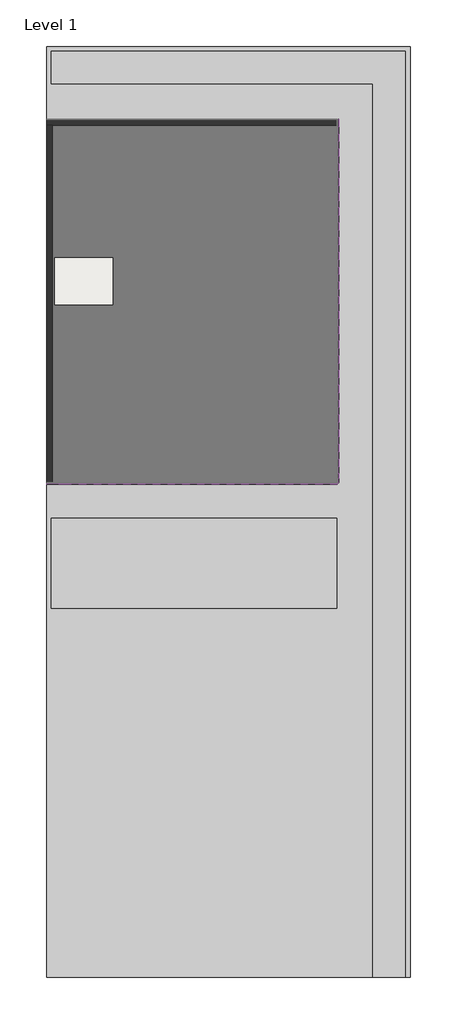
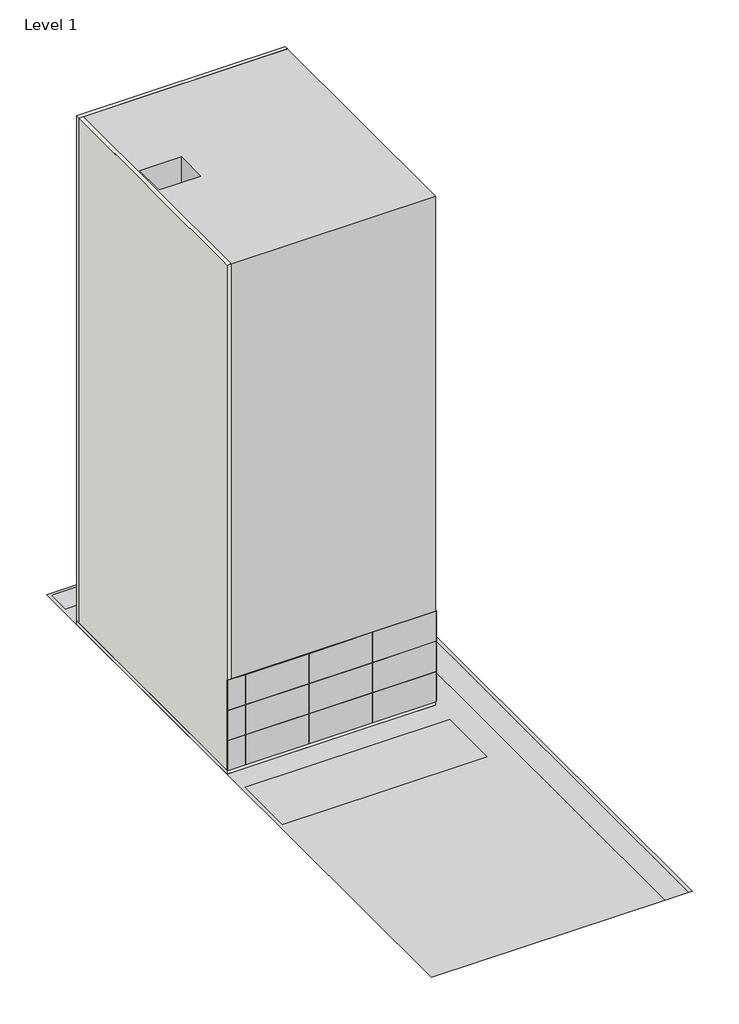
# One storey: 27 plates, 4 proxies, 2 walls, 1 slab.
"""IFC4 building model written with IfcOpenShell, lengths in millimetres."""

import ifcopenshell
import ifcopenshell.guid

model = None  # the IFC model being written
_history = None  # IfcOwnerHistory: only IFC2X3 demands one
_inside = {}  # id of a spatial element -> (the spatial element, [elements in it])
_under = {}  # id of a project, library or spatial element -> (it, [spatial elements below it])
_declared = {}  # id of a project -> (the project, [libraries it declares])
_typed = {}  # id of a type object -> (the type object, [elements of that type])
_made_of = {}  # id of a material, layer set ... -> (it, [elements and type objects made of it])


def new_model(schema):
    """Start an empty IFC model of exactly this schema.

    Asked for "IFC4X3", IfcOpenShell would pick the latest addendum, in which some entities
    have other attributes; the version numbers below select the first issue.
    IFC2X3 requires an IfcOwnerHistory on every rooted entity: one is made here for all.
    """
    global model, _history
    if schema == "IFC4X3":
        model = ifcopenshell.file(schema_version=(4, 3, 0, 0))
    else:
        model = ifcopenshell.file(schema=schema)
    _inside.clear()
    _under.clear()
    _declared.clear()
    _typed.clear()
    _made_of.clear()
    _history = None
    if model.schema == "IFC2X3":
        org = make("IfcOrganization", Name="unknown")
        user = make(
            "IfcPersonAndOrganization",
            ThePerson=make("IfcPerson", FamilyName="unknown"),
            TheOrganization=org,
        )
        app = make(
            "IfcApplication",
            ApplicationDeveloper=org,
            Version="unknown",
            ApplicationFullName="unknown",
            ApplicationIdentifier="unknown",
        )
        _history = make(
            "IfcOwnerHistory",
            OwningUser=user,
            OwningApplication=app,
            ChangeAction="ADDED",
            CreationDate=0,
        )
    return model


def make(cls, **values):
    """One entity of the class cls with the attributes given. An attribute that is None is left unset."""
    return model.create_entity(
        cls, **{name: value for name, value in values.items() if value is not None}
    )


def rooted(cls, **values):
    """An entity with a GlobalId (a new one), such as an element, a storey or a relation."""
    return make(cls, GlobalId=ifcopenshell.guid.new(), OwnerHistory=_history, **values)


def si_unit(unit_type, name, prefix=None):
    """IfcSIUnit, for example si_unit("LENGTHUNIT", "METRE", prefix="MILLI")."""
    return make("IfcSIUnit", UnitType=unit_type, Prefix=prefix, Name=name)


def assignment(units):
    """IfcUnitAssignment: the units of a project."""
    return None if units is None else make("IfcUnitAssignment", Units=units)


def point(xyz):
    """IfcCartesianPoint."""
    return None if xyz is None else make("IfcCartesianPoint", Coordinates=xyz)


def direction(xyz):
    """IfcDirection."""
    return None if xyz is None else make("IfcDirection", DirectionRatios=xyz)


def frame(location, z_axis=None, x_axis=None):
    """IfcAxis2Placement3D, a coordinate frame: its origin and axes. An axis left out is left unset."""
    return make(
        "IfcAxis2Placement3D",
        Location=point(location),
        Axis=direction(z_axis),
        RefDirection=direction(x_axis),
    )


def origin():
    """The frame at (0, 0, 0) with its axes left unset."""
    return frame((0.0, 0.0, 0.0))


def origin_with_axes():
    """The frame at (0, 0, 0) with the z axis (0, 0, 1) and the x axis (1, 0, 0) written out."""
    return frame((0.0, 0.0, 0.0), z_axis=(0.0, 0.0, 1.0), x_axis=(1.0, 0.0, 0.0))


def place(relative_to, where):
    """IfcLocalPlacement: puts the frame where relative to a parent placement (None: the world)."""
    return make(
        "IfcLocalPlacement", PlacementRelTo=relative_to, RelativePlacement=where
    )


def context(
    kind, dimensions, precision=None, world=None, true_north=None, identifier=None
):
    """IfcGeometricRepresentationContext, for example the 3D "Model" context."""
    return make(
        "IfcGeometricRepresentationContext",
        ContextIdentifier=identifier,
        ContextType=kind,
        CoordinateSpaceDimension=dimensions,
        Precision=precision,
        WorldCoordinateSystem=world,
        TrueNorth=true_north,
    )


def project(units=None, contexts=None):
    """IfcProject with its units and contexts."""
    return rooted(
        "IfcProject",
        Name="project",
        RepresentationContexts=contexts,
        UnitsInContext=assignment(units),
    )


def spatial(cls, under=None, at=None, **own):
    """A site, building, storey or space (cls), placed at a placement, below another one or the project."""
    s = rooted(cls, ObjectPlacement=at, **own)
    if under is not None:
        _under.setdefault(under.id(), (under, []))[1].append(s)
    return s


def polyline(points):
    """IfcPolyline through the points."""
    return make("IfcPolyline", Points=[point(p) for p in points])


def point_list(points):
    """IfcCartesianPointList2D or 3D."""
    cls = (
        "IfcCartesianPointList2D" if len(points[0]) == 2 else "IfcCartesianPointList3D"
    )
    return make(cls, CoordList=points)


def outline(outer, holes=None, kind="AREA"):
    """IfcArbitraryClosedProfileDef: a profile drawn as a closed curve; with holes, ...WithVoids."""
    if holes is None:
        return make("IfcArbitraryClosedProfileDef", ProfileType=kind, OuterCurve=outer)
    return make(
        "IfcArbitraryProfileDefWithVoids",
        ProfileType=kind,
        OuterCurve=outer,
        InnerCurves=holes,
    )


def extrude(swept, where, along, depth):
    """IfcExtrudedAreaSolid: the profile swept, set in the frame where, extruded along a direction by depth."""
    return make(
        "IfcExtrudedAreaSolid",
        SweptArea=swept,
        Position=where,
        ExtrudedDirection=direction(along),
        Depth=depth,
    )


def faces_of(points, faces, orient=None, outer=None):
    """IfcFace entities. A face is a list of loops; a loop is a list of indices into points, from 0.

    orient and outer hold one flag for each loop. By default every Orientation is true, the
    first loop of a face is its IfcFaceOuterBound and the others are IfcFaceBound.
    """
    made = []
    for i, loops in enumerate(faces):
        bounds = []
        for j, loop in enumerate(loops):
            is_outer = j == 0 if outer is None else outer[i][j]
            bounds.append(
                make(
                    "IfcFaceOuterBound" if is_outer else "IfcFaceBound",
                    Bound=make("IfcPolyLoop", Polygon=[points[k] for k in loop]),
                    Orientation=True if orient is None else orient[i][j],
                )
            )
        made.append(make("IfcFace", Bounds=bounds))
    return made


def faceted_brep(points, faces, orient=None, outer=None, voids=None):
    """IfcFacetedBrep: a solid bounded by flat faces; with voids (closed shells), ...WithVoids."""
    shared = [point(p) for p in points]
    hull = make("IfcClosedShell", CfsFaces=faces_of(shared, faces, orient, outer))
    if voids is None:
        return make("IfcFacetedBrep", Outer=hull)
    return make(
        "IfcFacetedBrepWithVoids",
        Outer=hull,
        Voids=[
            make(cls, CfsFaces=faces_of(shared, fs, o, b)) for cls, fs, o, b in voids
        ],
    )


def triangles(points, corners, closed=None, point_numbers=None):
    """IfcTriangulatedFaceSet: each triangle names its three corners, points numbered from 1."""
    return make(
        "IfcTriangulatedFaceSet",
        Coordinates=point_list(points),
        Closed=closed,
        CoordIndex=corners,
        PnIndex=point_numbers,
    )


def shape(context_of_items, identifier, shape_type, items):
    """IfcShapeRepresentation: the items that make up one representation, for example the "Body"."""
    return make(
        "IfcShapeRepresentation",
        ContextOfItems=context_of_items,
        RepresentationIdentifier=identifier,
        RepresentationType=shape_type,
        Items=items,
    )


def source(mapping_origin, context_of_items, identifier, shape_type, items):
    """IfcRepresentationMap: a shape defined once, which mapped items show again and again."""
    return make(
        "IfcRepresentationMap",
        MappingOrigin=mapping_origin,
        MappedRepresentation=shape(context_of_items, identifier, shape_type, items),
    )


def transform(
    local_origin,
    x_axis=None,
    y_axis=None,
    z_axis=None,
    scale=None,
    scale2=None,
    scale3=None,
    uniform=True,
):
    """IfcCartesianTransformationOperator3D, or its non-uniform kind. x_axis, y_axis, z_axis: its Axis1, 2, 3."""
    if uniform:
        return make(
            "IfcCartesianTransformationOperator3D",
            Axis1=direction(x_axis),
            Axis2=direction(y_axis),
            LocalOrigin=point(local_origin),
            Scale=scale,
            Axis3=direction(z_axis),
        )
    return make(
        "IfcCartesianTransformationOperator3DnonUniform",
        Axis1=direction(x_axis),
        Axis2=direction(y_axis),
        LocalOrigin=point(local_origin),
        Scale=scale,
        Axis3=direction(z_axis),
        Scale2=scale2,
        Scale3=scale3,
    )


def mapped(mapping_source, mapping_target):
    """IfcMappedItem: shows the shape of a source again, moved by a transform."""
    return make(
        "IfcMappedItem", MappingSource=mapping_source, MappingTarget=mapping_target
    )


def made_of(thing, what):
    """Note that an element or type object is made of a material, layer set ...; save() writes the relation."""
    if what is not None:
        _made_of.setdefault(what.id(), (what, []))[1].append(thing)
    return thing


def element(
    cls,
    number,
    at=None,
    inside=None,
    cuts=None,
    type_object=None,
    material=None,
    context=None,
    identifier="Body",
    shape_type=None,
    held_by="IfcProductDefinitionShape",
    body=None,
    shapes=None,
    **own,
):
    """One element of the class cls, such as IfcWall. Its Tag is "e" and its number.

    at: its placement. inside: the storey or other place that contains it. cuts: it is an
    opening in that element (IfcRelVoidsElement). A single representation is given by context,
    identifier, shape_type and body (its items); several are given by shapes. held_by: the class
    of the entity that holds the representations. save() writes the other relations.
    """
    e = rooted(cls, Tag="e%d" % number, ObjectPlacement=at, **own)
    if body is not None:
        shapes = [shape(context, identifier, shape_type, body)]
    if shapes is not None:
        e.Representation = make(held_by, Representations=shapes)
    if inside is not None:
        _inside.setdefault(inside.id(), (inside, []))[1].append(e)
    if cuts is not None:
        rooted(
            "IfcRelVoidsElement", RelatingBuildingElement=cuts, RelatedOpeningElement=e
        )
    if type_object is not None:
        _typed.setdefault(type_object.id(), (type_object, []))[1].append(e)
    return made_of(e, material)


def aggregate(whole, parts):
    """IfcRelAggregates: a whole, such as a stair, and the parts it consists of."""
    return rooted("IfcRelAggregates", RelatingObject=whole, RelatedObjects=parts)


def save(model, path):
    """Write the relations noted so far, then the file.

    IfcRelAggregates (storeys below a building ...), IfcRelContainedInSpatialStructure (elements
    in a storey), IfcRelDefinesByType, IfcRelAssociatesMaterial and IfcRelDeclares: one each for
    every whole, place, type object, material and project.
    """
    for whole, parts in _under.values():
        aggregate(whole, parts)
    for where, things in _inside.values():
        rooted(
            "IfcRelContainedInSpatialStructure",
            RelatedElements=things,
            RelatingStructure=where,
        )
    for kind, things in _typed.values():
        rooted("IfcRelDefinesByType", RelatedObjects=things, RelatingType=kind)
    for what, things in _made_of.values():
        rooted("IfcRelAssociatesMaterial", RelatedObjects=things, RelatingMaterial=what)
    for by, libraries in _declared.values():
        rooted("IfcRelDeclares", RelatingContext=by, RelatedDefinitions=libraries)
    model.write(path)


def system_panel_glazed_1e57f9bb(model_context):
    return source(origin(), model_context, "Body", "SweptSolid", [
        extrude(outline(polyline([(1524.0000002, 19.05), (-1524.0000002, 19.05), (-1524.0000002, 44.45), (1524.0000002, 44.45), (1524.0000002, 19.05)])), origin_with_axes(), (0.0, 0.0, 1.0), 1524.0),
    ])


def system_panel_glazed_ccfd9adb(model_context):
    return source(origin(), model_context, "Body", "SweptSolid", [
        extrude(outline(polyline([(427.9999998, 19.05), (-427.9999998, 19.05), (-427.9999998, 44.45), (427.9999998, 44.45), (427.9999998, 19.05)])), origin_with_axes(), (0.0, 0.0, 1.0), 1524.0),
    ])


def system_panel_glazed_88f24eba(model_context):
    return source(origin(), model_context, "Body", "SweptSolid", [
        extrude(outline(polyline([(153.9999998, 19.05), (-153.9999998, 19.05), (-153.9999998, 44.45), (153.9999998, 44.45), (153.9999998, 19.05)])), origin_with_axes(), (0.0, 0.0, 1.0), 1524.0),
    ])


model = new_model("IFC4")

# Units and contexts
model_context = context("Model", 3, world=origin())
ifc_project = project(units=[si_unit("LENGTHUNIT", "METRE", prefix="MILLI")], contexts=[model_context])

# Site, building, storey
site = spatial("IfcSite", under=ifc_project)
building = spatial("IfcBuilding", under=site)
storey = spatial("IfcBuildingStorey", under=building, Name="Level 1", Elevation=0.0)

# Proxies
placement = place(None, origin())
element("IfcBuildingElementProxy", 1, Name="Building Element Proxy", at=placement, inside=storey, context=model_context, shape_type="Tessellation", body=[
    triangles([(6161.6337845, 16399.6954926, -200.0000015), (-6338.3660202, 16399.6954926, -200.0000015), (-6338.3660202, 13899.6957642, -200.0000015), (3661.6340561, 13899.6957642, -200.0000015), (3661.6340561, 9999.6954437, -200.0000015), (3661.6340561, 1399.6955235, -200.0000015), (302.2590395, 1399.6955235, -200.0000015), (-6338.3660202, 1399.6955235, -200.0000015), (-6338.3660202, -15600.3047516, -200.0000015), (4861.6340652, -15600.3047516, -200.0000015), (4861.6340652, 13071.6951416, -200.0000015), (4861.6340652, 15099.6957733, -200.0000015), (-6188.3658737, 15099.6957733, -200.0000015), (-6188.3658737, 16249.6953461, -200.0000015), (6011.6342194, 16249.6953461, -200.0000015), (6011.6342194, 16015.6956757, -200.0000015), (6011.6342194, -15600.3047516, -200.0000015), (6161.6337845, -15600.3047516, -200.0000015), (3661.6340561, 199.695587, -200.0000015), (3661.6340561, -2920.304306, -200.0000015), (-1385.2410278, -2920.304306, -200.0000015), (-6188.3658737, -2920.304306, -200.0000015), (-6188.3658737, 199.695587, -200.0000015), (-166.490964, 199.695587, -200.0000015)], [[8, 9, 22], [22, 9, 21], [8, 22, 23], [24, 19, 7], [21, 9, 10], [23, 24, 8], [13, 2, 3], [13, 3, 4], [13, 14, 2], [13, 4, 12], [8, 24, 7], [2, 14, 1], [19, 6, 7], [11, 5, 6], [19, 20, 10], [16, 17, 18], [1, 16, 18], [20, 21, 10], [10, 11, 19], [4, 11, 12], [11, 4, 5], [16, 1, 15], [15, 1, 14], [19, 11, 6]], closed=False),
])
element("IfcBuildingElementProxy", 2, Name="Building Element Proxy", at=placement, inside=storey, context=model_context, shape_type="Tessellation", body=[
    triangles([(-6338.3660202, 1399.6955235, -200.1595303), (-6338.3660202, 1399.6955235, -200.0000015), (302.2590395, 1399.6955235, -200.1595303), (302.2590395, 1399.6955235, -200.0000015), (3661.6340561, 1399.6955235, -200.1595303), (3661.6340561, 1399.6955235, -200.0000015), (3661.6340561, 9999.6954437, -200.1595303), (3661.6340561, 9999.6954437, -200.0000015), (3661.6340561, 13899.6957642, -200.1595303), (3661.6340561, 13899.6957642, -200.0000015)], [[1, 4, 2], [1, 3, 4], [3, 6, 4], [3, 5, 6], [5, 8, 6], [5, 7, 8], [7, 10, 8], [7, 9, 10]], closed=False),
    triangles([(3661.6340561, 13899.6957642, -200.1595303), (3661.6340561, 13899.6957642, -200.0000015), (-6338.3660202, 13899.6957642, -200.1595303), (-6338.3660202, 13899.6957642, -200.0000015)], [[1, 4, 2], [1, 3, 4]], closed=False),
    triangles([(3661.6340561, 13899.6957642, -200.1595303), (-6338.3660202, 13899.6957642, -200.1595303), (-6338.3660202, 1399.6955235, -200.1595303), (3661.6340561, 1399.6955235, -200.1595303)], [[2, 3, 4], [4, 1, 2]], closed=False),
])
element("IfcBuildingElementProxy", 3, Name="Building Element Proxy", at=placement, inside=storey, context=model_context, shape_type="Tessellation", body=[
    triangles([(3661.6340561, 199.695587, -200.0000015), (-166.490964, 199.695587, -200.0000015), (-6188.3658737, 199.695587, -200.0000015), (-6188.3658737, -2920.304306, -200.0000015), (-1385.2410278, -2920.304306, -200.0000015), (3661.6340561, -2920.304306, -200.0000015), (6011.6342194, 16249.6953461, -200.0000015), (-6188.3658737, 16249.6953461, -200.0000015), (-6188.3658737, 15099.6957733, -200.0000015), (4861.6340652, 15099.6957733, -200.0000015), (4861.6340652, 13071.6951416, -200.0000015), (4861.6340652, -15600.3047516, -200.0000015), (6011.6342194, -15600.3047516, -200.0000015), (6011.6342194, 16015.6956757, -200.0000015)], [[4, 5, 3], [3, 5, 2], [10, 8, 9], [6, 1, 2], [2, 5, 6], [12, 13, 11], [14, 11, 13], [10, 11, 14], [14, 7, 10], [10, 7, 8]], closed=False),
])
element("IfcBuildingElementProxy", 4, Name="Ed. 8 pavimentos : Ed. 8 pavimentos", ObjectType="Ed. 8 pavimentos : Ed. 8 pavimentos", at=placement, inside=storey, context=model_context, shape_type="SweptSolid", body=[
    extrude(outline(polyline([(-6338.3659636, 13899.6955828), (3661.6340364, 13899.6955828), (3661.6340364, 1399.6955828), (-6338.3659636, 1399.6955828), (-6338.3659636, 13899.6955828)]), holes=[polyline([(-4062.8993101, 9130.9023719), (-6062.8993101, 9130.9023719), (-6062.8993101, 7530.9023719), (-4062.8993101, 7530.9023719), (-4062.8993101, 9130.9023719)])]), origin_with_axes(), (0.0, 0.0, 1.0), 25600.0),
])

# Plates
system_panel_glazed_shape = system_panel_glazed_1e57f9bb(model_context)
element("IfcPlate", 5, ObjectType="System Panel : Glazed", at=placement, inside=storey, context=model_context, shape_type="MappedRepresentation", body=[
    mapped(system_panel_glazed_shape, transform((2137.6340362, 1399.6955828, 0.0), x_axis=(-1.0, 0.0, 0.0), y_axis=(0.0, -1.0, 0.0), z_axis=(0.0, 0.0, 1.0))),
])
element("IfcPlate", 6, ObjectType="System Panel : Glazed", at=placement, inside=storey, context=model_context, shape_type="MappedRepresentation", body=[
    mapped(system_panel_glazed_shape, transform((3661.6340364, 12375.6955827, 0.0), x_axis=(0.0, -1.0, 0.0), y_axis=(1.0, 0.0, 0.0), z_axis=(0.0, 0.0, 1.0))),
])
element("IfcPlate", 7, ObjectType="System Panel : Glazed", at=placement, inside=storey, context=model_context, shape_type="MappedRepresentation", body=[
    mapped(system_panel_glazed_shape, transform((-910.3659639, 1399.6955828, 0.0), x_axis=(-1.0, 0.0, 0.0), y_axis=(0.0, -1.0, 0.0), z_axis=(0.0, 0.0, 1.0))),
])
element("IfcPlate", 8, ObjectType="System Panel : Glazed", at=placement, inside=storey, context=model_context, shape_type="MappedRepresentation", body=[
    mapped(system_panel_glazed_shape, transform((-3958.3659639, 1399.6955828, 0.0), x_axis=(-1.0, 0.0, 0.0), y_axis=(0.0, -1.0, 0.0), z_axis=(0.0, 0.0, 1.0))),
])
element("IfcPlate", 9, ObjectType="System Panel : Glazed", at=placement, inside=storey, context=model_context, shape_type="MappedRepresentation", body=[
    mapped(system_panel_glazed_shape, transform((2137.6340362, 1399.6955828, 1524.0), x_axis=(-1.0, 0.0, 0.0), y_axis=(0.0, -1.0, 0.0), z_axis=(0.0, 0.0, 1.0))),
])
element("IfcPlate", 10, ObjectType="System Panel : Glazed", at=placement, inside=storey, context=model_context, shape_type="MappedRepresentation", body=[
    mapped(system_panel_glazed_shape, transform((-910.3659639, 1399.6955828, 1524.0), x_axis=(-1.0, 0.0, 0.0), y_axis=(0.0, -1.0, 0.0), z_axis=(0.0, 0.0, 1.0))),
])
element("IfcPlate", 11, ObjectType="System Panel : Glazed", at=placement, inside=storey, context=model_context, shape_type="MappedRepresentation", body=[
    mapped(system_panel_glazed_shape, transform((-3958.3659639, 1399.6955828, 1524.0), x_axis=(-1.0, 0.0, 0.0), y_axis=(0.0, -1.0, 0.0), z_axis=(0.0, 0.0, 1.0))),
])
element("IfcPlate", 12, ObjectType="System Panel : Glazed", at=placement, inside=storey, context=model_context, shape_type="MappedRepresentation", body=[
    mapped(system_panel_glazed_shape, transform((2137.6340362, 1399.6955828, 3048.0), x_axis=(-1.0, 0.0, 0.0), y_axis=(0.0, -1.0, 0.0), z_axis=(0.0, 0.0, 1.0))),
])
element("IfcPlate", 13, ObjectType="System Panel : Glazed", at=placement, inside=storey, context=model_context, shape_type="MappedRepresentation", body=[
    mapped(system_panel_glazed_shape, transform((-910.3659639, 1399.6955828, 3048.0), x_axis=(-1.0, 0.0, 0.0), y_axis=(0.0, -1.0, 0.0), z_axis=(0.0, 0.0, 1.0))),
])
element("IfcPlate", 14, ObjectType="System Panel : Glazed", at=placement, inside=storey, context=model_context, shape_type="MappedRepresentation", body=[
    mapped(system_panel_glazed_shape, transform((-3958.3659639, 1399.6955828, 3048.0), x_axis=(-1.0, 0.0, 0.0), y_axis=(0.0, -1.0, 0.0), z_axis=(0.0, 0.0, 1.0))),
])
element("IfcPlate", 15, ObjectType="System Panel : Glazed", at=placement, inside=storey, context=model_context, shape_type="MappedRepresentation", body=[
    mapped(system_panel_glazed_shape, transform((3661.6340364, 9327.6955825, 0.0), x_axis=(0.0, -1.0, 0.0), y_axis=(1.0, 0.0, 0.0), z_axis=(0.0, 0.0, 1.0))),
])
element("IfcPlate", 16, ObjectType="System Panel : Glazed", at=placement, inside=storey, context=model_context, shape_type="MappedRepresentation", body=[
    mapped(system_panel_glazed_shape, transform((3661.6340364, 6279.6955825, 0.0), x_axis=(0.0, -1.0, 0.0), y_axis=(1.0, 0.0, 0.0), z_axis=(0.0, 0.0, 1.0))),
])
element("IfcPlate", 17, ObjectType="System Panel : Glazed", at=placement, inside=storey, context=model_context, shape_type="MappedRepresentation", body=[
    mapped(system_panel_glazed_shape, transform((3661.6340364, 3231.6955825, 0.0), x_axis=(0.0, -1.0, 0.0), y_axis=(1.0, 0.0, 0.0), z_axis=(0.0, 0.0, 1.0))),
])
element("IfcPlate", 18, ObjectType="System Panel : Glazed", at=placement, inside=storey, context=model_context, shape_type="MappedRepresentation", body=[
    mapped(system_panel_glazed_shape, transform((3661.6340364, 12375.6955827, 1524.0), x_axis=(0.0, -1.0, 0.0), y_axis=(1.0, 0.0, 0.0), z_axis=(0.0, 0.0, 1.0))),
])
element("IfcPlate", 19, ObjectType="System Panel : Glazed", at=placement, inside=storey, context=model_context, shape_type="MappedRepresentation", body=[
    mapped(system_panel_glazed_shape, transform((3661.6340364, 9327.6955825, 1524.0), x_axis=(0.0, -1.0, 0.0), y_axis=(1.0, 0.0, 0.0), z_axis=(0.0, 0.0, 1.0))),
])
element("IfcPlate", 20, ObjectType="System Panel : Glazed", at=placement, inside=storey, context=model_context, shape_type="MappedRepresentation", body=[
    mapped(system_panel_glazed_shape, transform((3661.6340364, 6279.6955825, 1524.0), x_axis=(0.0, -1.0, 0.0), y_axis=(1.0, 0.0, 0.0), z_axis=(0.0, 0.0, 1.0))),
])
element("IfcPlate", 21, ObjectType="System Panel : Glazed", at=placement, inside=storey, context=model_context, shape_type="MappedRepresentation", body=[
    mapped(system_panel_glazed_shape, transform((3661.6340364, 3231.6955825, 1524.0), x_axis=(0.0, -1.0, 0.0), y_axis=(1.0, 0.0, 0.0), z_axis=(0.0, 0.0, 1.0))),
])
element("IfcPlate", 22, ObjectType="System Panel : Glazed", at=placement, inside=storey, context=model_context, shape_type="MappedRepresentation", body=[
    mapped(system_panel_glazed_shape, transform((3661.6340364, 12375.6955827, 3048.0), x_axis=(0.0, -1.0, 0.0), y_axis=(1.0, 0.0, 0.0), z_axis=(0.0, 0.0, 1.0))),
])
element("IfcPlate", 23, ObjectType="System Panel : Glazed", at=placement, inside=storey, context=model_context, shape_type="MappedRepresentation", body=[
    mapped(system_panel_glazed_shape, transform((3661.6340364, 9327.6955825, 3048.0), x_axis=(0.0, -1.0, 0.0), y_axis=(1.0, 0.0, 0.0), z_axis=(0.0, 0.0, 1.0))),
])
element("IfcPlate", 24, ObjectType="System Panel : Glazed", at=placement, inside=storey, context=model_context, shape_type="MappedRepresentation", body=[
    mapped(system_panel_glazed_shape, transform((3661.6340364, 6279.6955825, 3048.0), x_axis=(0.0, -1.0, 0.0), y_axis=(1.0, 0.0, 0.0), z_axis=(0.0, 0.0, 1.0))),
])
element("IfcPlate", 25, ObjectType="System Panel : Glazed", at=placement, inside=storey, context=model_context, shape_type="MappedRepresentation", body=[
    mapped(system_panel_glazed_shape, transform((3661.6340364, 3231.6955825, 3048.0), x_axis=(0.0, -1.0, 0.0), y_axis=(1.0, 0.0, 0.0), z_axis=(0.0, 0.0, 1.0))),
])
system_panel_glazed_2_shape = system_panel_glazed_ccfd9adb(model_context)
element("IfcPlate", 26, ObjectType="System Panel : Glazed", at=placement, inside=storey, context=model_context, shape_type="MappedRepresentation", body=[
    mapped(system_panel_glazed_2_shape, transform((-5910.3659638, 1399.6955828, 0.0), x_axis=(-1.0, 0.0, 0.0), y_axis=(0.0, -1.0, 0.0), z_axis=(0.0, 0.0, 1.0))),
])
element("IfcPlate", 27, ObjectType="System Panel : Glazed", at=placement, inside=storey, context=model_context, shape_type="MappedRepresentation", body=[
    mapped(system_panel_glazed_2_shape, transform((-5910.3659638, 1399.6955828, 1524.0), x_axis=(-1.0, 0.0, 0.0), y_axis=(0.0, -1.0, 0.0), z_axis=(0.0, 0.0, 1.0))),
])
element("IfcPlate", 28, ObjectType="System Panel : Glazed", at=placement, inside=storey, context=model_context, shape_type="MappedRepresentation", body=[
    mapped(system_panel_glazed_2_shape, transform((-5910.3659638, 1399.6955828, 3048.0), x_axis=(-1.0, 0.0, 0.0), y_axis=(0.0, -1.0, 0.0), z_axis=(0.0, 0.0, 1.0))),
])
system_panel_glazed_3_shape = system_panel_glazed_88f24eba(model_context)
element("IfcPlate", 29, ObjectType="System Panel : Glazed", at=placement, inside=storey, context=model_context, shape_type="MappedRepresentation", body=[
    mapped(system_panel_glazed_3_shape, transform((3661.6340364, 1553.6955827, 0.0), x_axis=(0.0, -1.0, 0.0), y_axis=(1.0, 0.0, 0.0), z_axis=(0.0, 0.0, 1.0))),
])
element("IfcPlate", 30, ObjectType="System Panel : Glazed", at=placement, inside=storey, context=model_context, shape_type="MappedRepresentation", body=[
    mapped(system_panel_glazed_3_shape, transform((3661.6340364, 1553.6955827, 1524.0), x_axis=(0.0, -1.0, 0.0), y_axis=(1.0, 0.0, 0.0), z_axis=(0.0, 0.0, 1.0))),
])
element("IfcPlate", 31, ObjectType="System Panel : Glazed", at=placement, inside=storey, context=model_context, shape_type="MappedRepresentation", body=[
    mapped(system_panel_glazed_3_shape, transform((3661.6340364, 1553.6955827, 3048.0), x_axis=(0.0, -1.0, 0.0), y_axis=(1.0, 0.0, 0.0), z_axis=(0.0, 0.0, 1.0))),
])

# Slab
element("IfcSlab", 32, ObjectType="Plataforma - concreto magro", at=placement, inside=storey, context=model_context, shape_type="SweptSolid", body=[
    extrude(outline(polyline([(3661.6340364, 13899.6955828), (3661.6340364, 1399.6955828), (-6338.3659636, 1399.6955828), (-6338.3659636, 13899.6955828), (3661.6340364, 13899.6955828)])), frame((0.0, 0.0, -200.0), z_axis=(0.0, 0.0, 1.0), x_axis=(1.0, 0.0, 0.0)), (0.0, 0.0, 1.0), 200.0),
])

# Walls
element("IfcWall", 33, ObjectType="Generic - 8\"", at=placement, inside=storey, context=model_context, shape_type="Brep", body=[
    faceted_brep([(3661.6340364, 13899.6955828, 0.0), (-6338.3659636, 13899.6955828, 0.0), (-6338.3659636, 13899.6955828, 25600.0), (3661.6340364, 13899.6955828, 25600.0), (3661.6340364, 13696.4955828, 0.0), (3661.6340364, 13696.4955828, 25600.0), (-6135.1659636, 13696.4955828, 25600.0), (-6338.3659636, 13696.4955828, 25600.0), (-6338.3659636, 13696.4955828, 0.0), (-6135.1659636, 13696.4955828, 0.0)], [[[0, 1, 2, 3]], [[4, 5, 6, 7, 8, 9]], [[1, 0, 4, 9, 8]], [[3, 2, 7, 6, 5]], [[0, 3, 5, 4]], [[2, 1, 8, 7]]]),
])
element("IfcWall", 34, ObjectType="Generic - 8\"", at=placement, inside=storey, context=model_context, shape_type="SweptSolid", body=[
    extrude(outline(polyline([(-6338.3659636, 1399.6955828), (-6338.3659636, 13696.4955828), (-6135.1659636, 13696.4955828), (-6135.1659636, 1399.6955828), (-6338.3659636, 1399.6955828)])), origin_with_axes(), (0.0, 0.0, 1.0), 25600.0),
])

save(model, "model.ifc")

# Revit data of these elements
# Project information
#   Project Issue Date = "Issue Date"
#   Project Status = "Project Status"
#   Client Name = "Owner"
#   Project Address = "Enter address here"
#   Project Name = "Project Name"
#   Project Number = "Project Number"
# Type "System Panel : Glazed"
#   Construction Type Id = "GSP4R"
#   Analytic Construction = "1/8 in Pilkington single glazing"
#   Visual Light Transmittance = 0.9
#   Solar Heat Gain Coefficient = 0.86
#   Heat Transfer Coefficient (U) = 6.7069 W/(m²·K)
# Type "Plataforma - concreto magro"
#   Layers, outside or top first: 0.20 m "Concrete, Precast" (function 1)
# Type "Generic - 8\""
#   Assembly Code = "B2010"
#   Layers, outside or top first: 0.2032 m no material (function 1)
# Elements 1, 2 (IfcBuildingElementProxy)
#   Material = none
#   Phase Created = New Construction
# Element 3 (IfcBuildingElementProxy)
#   Material = _grama
#   Phase Created = New Construction
# Element 4 (IfcBuildingElementProxy, "Ed. 8 pavimentos : Ed. 8 pavimentos")
#   Phase Created = New Construction
#   Materials on its faces: "Default Form"
# Elements 5, 6, 7, 8, 9, 10, 11, 12, 13, 14, 15, 16, 17, 18, 19, 20, 21, 22, 23, 24, 25, 26, 27, 28, 29, 30, 31 (IfcPlate, "System Panel : Glazed")
#   Phase Created = New Construction
#   Materials on its faces: "Glass"
# Element 32 (IfcSlab, "Plataforma - concreto magro")
#   Phase Created = New Construction
#   Materials on its faces: "Concrete, Precast"
# Elements 33, 34 (IfcWall, "Generic - 8\"")
#   Top Offset = 0.00 m
#   Base Offset = 0.00 m
#   Unconnected Height = 25.60 m
#   wall height = 25.60 m
#   Phase Created = New Construction
#   Base Constraint = Level 1
#   Materials on its faces: "Default Wall"
# Materials
#   "Concrete, Precast": class "Concrete", colour RGB 198 187 187, transparency 0, Description = "Precast concrete", Cost = 0
#   "_grama": class "Generic", colour RGB 87 117 55, transparency 0, Cost = 0
#   "Default Form": class "Generic", colour RGB 185 189 196, transparency 0.5, Cost = 0
#   "Glass": class "Glass", colour RGB 0 128 192, transparency 0.75, Description = "Soda Lime Glass", Cost = 0
#   "Default Wall": class "Miscellaneous", colour RGB 128 128 128, transparency 0, Cost = 0
